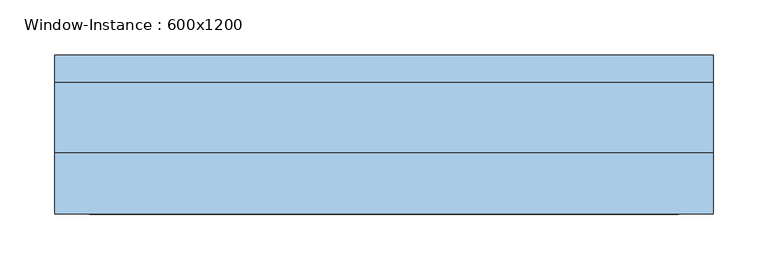
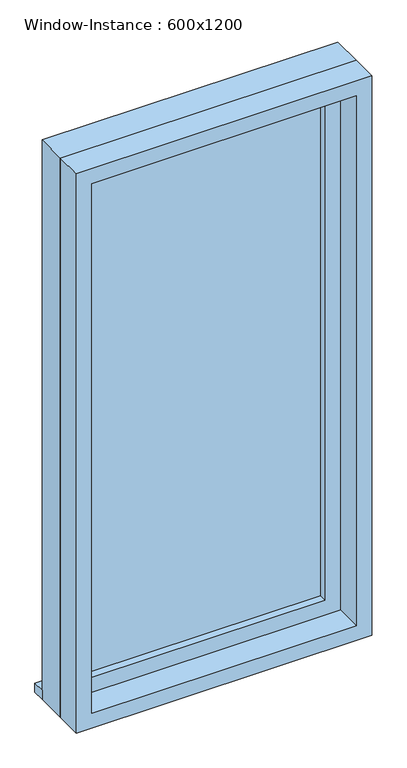
"""IFC4 building model written with IfcOpenShell, lengths in millimetres: window geometry, Window-Instance : 600x1200."""

from ifc_helpers import new_model, si_unit, frame, origin, place, context, project, spatial, polyline, outline, extrude, source, transform, mapped, element, save


def window_instance_600x1200_d180a32f(model_context):
    return source(origin(), model_context, "Body", "SweptSolid", [
        extrude(outline(polyline([(-338.1, 85.4), (261.9, 85.4), (261.9, 60.0), (-338.1, 60.0), (-338.1, 85.4)])), frame((0.0, 0.0, 900.0), z_axis=(0.0, 0.0, 1.0), x_axis=(1.0, 0.0, 0.0)), (0.0, 0.0, 1.0), 19.05),
        extrude(outline(polyline([(198.4, 11.425), (-274.6, 11.425), (-274.6, 24.125), (198.4, 24.125), (198.4, 11.425)])), frame((0.0, 0.0, 963.5), z_axis=(0.0, 0.0, 1.0), x_axis=(1.0, 0.0, 0.0)), (0.0, 0.0, 1.0), 1073.0),
        extrude(outline(polyline([(2080.95, -319.05), (919.05, -319.05), (919.05, 242.85), (2080.95, 242.85), (2080.95, -319.05)]), holes=[polyline([(2036.5, -274.6), (2036.5, 198.4), (963.5, 198.4), (963.5, -274.6), (2036.5, -274.6)])]), frame((0.0, -4.45, 0.0), z_axis=(0.0, 1.0, 0.0), x_axis=(0.0, 0.0, 1.0)), (0.0, 0.0, 1.0), 44.45),
        extrude(outline(polyline([(2100.0, -338.1), (900.0, -338.1), (900.0, 261.9), (2100.0, 261.9), (2100.0, -338.1)]), holes=[polyline([(2068.25, -306.35), (2068.25, 230.15), (931.75, 230.15), (931.75, -306.35), (2068.25, -306.35)])]), frame((0.0, -60.0, 0.0), z_axis=(0.0, 1.0, 0.0), x_axis=(0.0, 0.0, 1.0)), (0.0, 0.0, 1.0), 55.55),
        extrude(outline(polyline([(2100.0, 261.9), (2100.0, -338.1), (900.0, -338.1), (900.0, 261.9), (2100.0, 261.9)]), holes=[polyline([(2080.95, 242.85), (919.05, 242.85), (919.05, -319.05), (2080.95, -319.05), (2080.95, 242.85)])]), frame((0.0, -4.45, 0.0), z_axis=(0.0, 1.0, 0.0), x_axis=(0.0, 0.0, 1.0)), (0.0, 0.0, 1.0), 64.45),
    ])


if __name__ == "__main__":
    model = new_model("IFC4")
    model_context = context("Model", 3, world=origin())
    ifc_project = project(units=[si_unit("LENGTHUNIT", "METRE", prefix="MILLI")], contexts=[model_context])
    site = spatial("IfcSite", under=ifc_project)
    building = spatial("IfcBuilding", under=site)
    placement = place(None, origin())
    window_instance_600x1200_shape = window_instance_600x1200_d180a32f(model_context)
    element("IfcWindow", 1, ObjectType="Window-Instance : 600x1200", at=placement, inside=building, context=model_context, shape_type="MappedRepresentation", body=[
        mapped(window_instance_600x1200_shape, transform((0.0, 0.0, 0.0), x_axis=(1.0, 0.0, 0.0), y_axis=(0.0, 1.0, 0.0), z_axis=(0.0, 0.0, 1.0))),
    ])
    save(model, "model.ifc")

# Revit data of these elements
# Type "Window-Instance : 600x1200"
#   Type Mark = "7"
#   Construction Type Id = "GSP4R"
#   Assembly Code = "B2020100"
#   Analytic Construction = "1/8 in Pilkington single glazing"
#   Visual Light Transmittance = 0.9
#   Thermal Resistance (R) = 0.149095 (m²·K)/W
#   Solar Heat Gain Coefficient = 0.86
#   Heat Transfer Coefficient (U) = 6.70716 W/(m²·K)
#   Height [instance default] = 1200 mm
#   Default Sill Height = 900 mm
#   Width [instance default] = 600 mm
#   Window Inset = 20 mm
#   Glass Pane Material = WW-EC-GL-Storefront
#   Sash Material = WW-EC-RGB-White
#   Wall Closure = (empty or 0)
# Element 1 (IfcWindow, "Window-Instance : 600x1200")
#   Materials on its faces: "WW-EC-RGB-White", "WW-EC-GL-Storefront"
# Materials
#   "WW-EC-GL-Storefront": class "Glass", colour RGB 236 240 239, transparency 0.85, Description = "Storefront Glass", Cost = 0
#   "WW-EC-RGB-White": class "Generic", colour RGB 255 255 255, transparency 0, Comments = "If region requests off-white, swith asset color to RGB 231-228-220", Description = "Generic Color", Cost = 0
